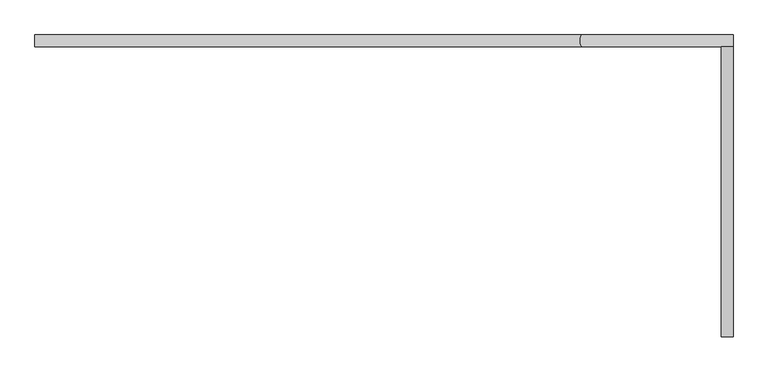
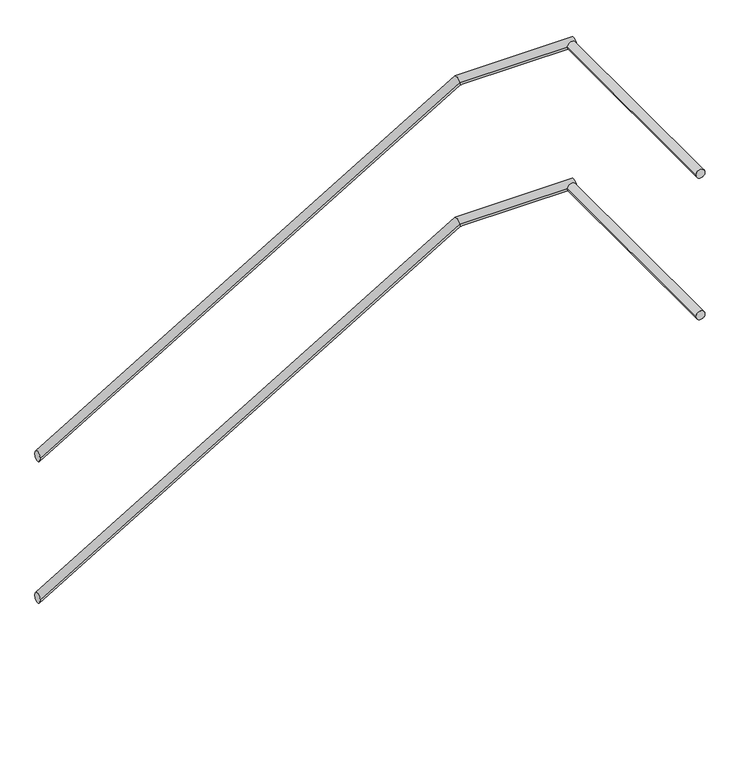
"""IFC4 building model written with IfcOpenShell, lengths in millimetres: railing geometry."""

from ifc_helpers import new_model, si_unit, frame, origin, place, context, project, spatial, circle_curve, ellipse_curve, source, transform, mapped, element, save
from ifc_brep_helpers import plane_surface, cylinder_surface, advanced_brep


def railing_5d0a0082(model_context):
    return source(origin(), model_context, "Body", "AdvancedBrep", [
        advanced_brep(
        [(43964.6, 23749.5208589, 1734.9618634), (43994.6, 23749.5208589, 1734.9618634), (43964.6, 24494.1208589, 1734.9618634), (43994.6, 24494.1208589, 1734.9618634)],
        [
            (0, 1, circle_curve(frame((43979.6, 23749.5208589, 1734.9618634), z_axis=(0.0, -1.0, 0.0), x_axis=(1.0, 0.0, 0.0)), 15.0)),
            (1, 0, circle_curve(frame((43979.6, 23749.5208589, 1734.9618634), z_axis=(0.0, -1.0, 0.0), x_axis=(1.0, 0.0, 0.0)), 15.0)),
            (2, 3, circle_curve(frame((43979.6, 24494.1208589, 1734.9618634), z_axis=(0.0, 1.0, 0.0), x_axis=(1.0, 0.0, 0.0)), 15.0)),
            (3, 2, circle_curve(frame((43979.6, 24494.1208589, 1734.9618634), z_axis=(0.0, 1.0, 0.0), x_axis=(1.0, 0.0, 0.0)), 15.0)),
            (0, 2),
            (3, 1),
        ],
        [
            plane_surface(frame((43979.6, 23749.5208589, 1749.9618634), z_axis=(0.0, -1.0, 0.0), x_axis=(0.0, 0.0, 1.0))),
            plane_surface(frame((43979.6, 24494.1208589, 1749.9618634), z_axis=(0.0, 1.0, 0.0), x_axis=(0.0, 0.0, 1.0))),
            cylinder_surface(frame((43979.6, 23749.5208589, 1734.9618634), z_axis=(0.0, -1.0, 0.0), x_axis=(1.0, 0.0, 0.0)), 15.0),
        ],
        [
            (0, [[1, 2]]),
            (1, [[3, 4]]),
            (2, [[-1, 5, -4, 6]]),
            (2, [[-2, -6, -3, -5]]),
        ],
    ),
        advanced_brep(
        [(43994.6, 24494.1208589, 1734.9618634), (43994.6, 24524.1208589, 1734.9618634), (43606.242552, 24494.1208589, 1734.9618634), (43606.242552, 24524.1208589, 1734.9618634), (42202.1161135, 24494.1208589, 899.1723166), (42202.1161135, 24524.1208589, 899.1723166)],
        [
            (0, 1, circle_curve(frame((43994.6, 24509.1208589, 1734.9618634), z_axis=(1.0, 0.0, 0.0), x_axis=(0.0, 1.0, 0.0)), 15.0)),
            (1, 0, circle_curve(frame((43994.6, 24509.1208589, 1734.9618634), z_axis=(1.0, 0.0, 0.0), x_axis=(0.0, 1.0, 0.0)), 15.0)),
            (0, 2),
            (2, 3, ellipse_curve(frame((43606.242552, 24509.1208589, 1734.9618634), z_axis=(0.9641817474962143, 0.0, 0.26524245096731114), x_axis=(0.265242450967311, 0.0, -0.9641817474962145)), 15.5572329, 15.0)),
            (3, 1),
            (3, 2, ellipse_curve(frame((43606.242552, 24509.1208589, 1734.9618634), z_axis=(0.9641817474962143, 0.0, 0.26524245096731114), x_axis=(0.265242450967311, 0.0, -0.9641817474962145)), 15.5572329, 15.0)),
            (4, 5, ellipse_curve(frame((42202.1161135, 24509.1208589, 899.1723166), z_axis=(-1.0, 0.0, 0.0), x_axis=(0.0, 0.0, 1.0)), 17.4562134, 15.0)),
            (5, 4, ellipse_curve(frame((42202.1161135, 24509.1208589, 899.1723166), z_axis=(-1.0, 0.0, 0.0), x_axis=(0.0, 0.0, 1.0)), 17.4562134, 15.0)),
            (2, 4),
            (5, 3),
        ],
        [
            plane_surface(frame((43994.6, 24509.1208589, 1749.9618634), z_axis=(1.0, 0.0, 0.0), x_axis=(0.0, -1.0, 0.0))),
            cylinder_surface(frame((43994.6, 24509.1208589, 1734.9618634), z_axis=(1.0, 0.0, 0.0), x_axis=(0.0, 1.0, 0.0)), 15.0),
            plane_surface(frame((42202.1161135, 24509.1208589, 916.62853), z_axis=(-1.0, 0.0, 0.0), x_axis=(0.0, -1.0, 0.0))),
            cylinder_surface(frame((43609.7883714, 24509.1208589, 1737.0724701), z_axis=(0.8592928844097072, 0.0, 0.511483859767682), x_axis=(0.0, 1.0, 0.0)), 15.0),
        ],
        [
            (0, [[1, 2]]),
            (1, [[-1, 3, 4, 5]]),
            (1, [[-2, -5, 6, -3]]),
            (2, [[7, 8]]),
            (3, [[-4, 9, -8, 10]]),
            (3, [[-6, -10, -7, -9]]),
        ],
    ),
        advanced_brep(
        [(43964.6, 23749.5208589, 2234.9618634), (43994.6, 23749.5208589, 2234.9618634), (43964.6, 24494.1208589, 2234.9618634), (43994.6, 24494.1208589, 2234.9618634)],
        [
            (0, 1, circle_curve(frame((43979.6, 23749.5208589, 2234.9618634), z_axis=(0.0, -1.0, 0.0), x_axis=(1.0, 0.0, 0.0)), 15.0)),
            (1, 0, circle_curve(frame((43979.6, 23749.5208589, 2234.9618634), z_axis=(0.0, -1.0, 0.0), x_axis=(1.0, 0.0, 0.0)), 15.0)),
            (2, 3, circle_curve(frame((43979.6, 24494.1208589, 2234.9618634), z_axis=(0.0, 1.0, 0.0), x_axis=(1.0, 0.0, 0.0)), 15.0)),
            (3, 2, circle_curve(frame((43979.6, 24494.1208589, 2234.9618634), z_axis=(0.0, 1.0, 0.0), x_axis=(1.0, 0.0, 0.0)), 15.0)),
            (0, 2),
            (3, 1),
        ],
        [
            plane_surface(frame((43979.6, 23749.5208589, 2249.9618634), z_axis=(0.0, -1.0, 0.0), x_axis=(0.0, 0.0, 1.0))),
            plane_surface(frame((43979.6, 24494.1208589, 2249.9618634), z_axis=(0.0, 1.0, 0.0), x_axis=(0.0, 0.0, 1.0))),
            cylinder_surface(frame((43979.6, 23749.5208589, 2234.9618634), z_axis=(0.0, -1.0, 0.0), x_axis=(1.0, 0.0, 0.0)), 15.0),
        ],
        [
            (0, [[1, 2]]),
            (1, [[3, 4]]),
            (2, [[-1, 5, -4, 6]]),
            (2, [[-2, -6, -3, -5]]),
        ],
    ),
        advanced_brep(
        [(43994.6, 24494.1208589, 2234.9618634), (43994.6, 24524.1208589, 2234.9618634), (43606.242552, 24494.1208589, 2234.9618634), (43606.242552, 24524.1208589, 2234.9618634), (42202.1161135, 24494.1208589, 1399.1723166), (42202.1161135, 24524.1208589, 1399.1723166)],
        [
            (0, 1, circle_curve(frame((43994.6, 24509.1208589, 2234.9618634), z_axis=(1.0, 0.0, 0.0), x_axis=(0.0, 1.0, 0.0)), 15.0)),
            (1, 0, circle_curve(frame((43994.6, 24509.1208589, 2234.9618634), z_axis=(1.0, 0.0, 0.0), x_axis=(0.0, 1.0, 0.0)), 15.0)),
            (0, 2),
            (2, 3, ellipse_curve(frame((43606.242552, 24509.1208589, 2234.9618634), z_axis=(0.9641817474962143, 0.0, 0.26524245096731114), x_axis=(0.265242450967311, 0.0, -0.9641817474962145)), 15.5572329, 15.0)),
            (3, 1),
            (3, 2, ellipse_curve(frame((43606.242552, 24509.1208589, 2234.9618634), z_axis=(0.9641817474962143, 0.0, 0.26524245096731114), x_axis=(0.265242450967311, 0.0, -0.9641817474962145)), 15.5572329, 15.0)),
            (4, 5, ellipse_curve(frame((42202.1161135, 24509.1208589, 1399.1723166), z_axis=(-1.0, 0.0, 0.0), x_axis=(0.0, 0.0, 1.0)), 17.4562134, 15.0)),
            (5, 4, ellipse_curve(frame((42202.1161135, 24509.1208589, 1399.1723166), z_axis=(-1.0, 0.0, 0.0), x_axis=(0.0, 0.0, 1.0)), 17.4562134, 15.0)),
            (2, 4),
            (5, 3),
        ],
        [
            plane_surface(frame((43994.6, 24509.1208589, 2249.9618634), z_axis=(1.0, 0.0, 0.0), x_axis=(0.0, -1.0, 0.0))),
            cylinder_surface(frame((43994.6, 24509.1208589, 2234.9618634), z_axis=(1.0, 0.0, 0.0), x_axis=(0.0, 1.0, 0.0)), 15.0),
            plane_surface(frame((42202.1161135, 24509.1208589, 1416.62853), z_axis=(-1.0, 0.0, 0.0), x_axis=(0.0, -1.0, 0.0))),
            cylinder_surface(frame((43609.7883714, 24509.1208589, 2237.0724701), z_axis=(0.8592928844097072, 0.0, 0.511483859767682), x_axis=(0.0, 1.0, 0.0)), 15.0),
        ],
        [
            (0, [[1, 2]]),
            (1, [[-1, 3, 4, 5]]),
            (1, [[-2, -5, 6, -3]]),
            (2, [[7, 8]]),
            (3, [[-4, 9, -8, 10]]),
            (3, [[-6, -10, -7, -9]]),
        ],
    ),
    ])


if __name__ == "__main__":
    model = new_model("IFC4")
    model_context = context("Model", 3, world=origin())
    ifc_project = project(units=[si_unit("LENGTHUNIT", "METRE", prefix="MILLI")], contexts=[model_context])
    site = spatial("IfcSite", under=ifc_project)
    building = spatial("IfcBuilding", under=site)
    placement = place(None, origin())
    railing_shape = railing_5d0a0082(model_context)
    element("IfcRailing", 1, at=placement, inside=building, context=model_context, shape_type="MappedRepresentation", body=[
        mapped(railing_shape, transform((0.0, 0.0, 0.0), x_axis=(1.0, 0.0, 0.0), y_axis=(0.0, 1.0, 0.0), z_axis=(0.0, 0.0, 1.0))),
    ])
    save(model, "model.ifc")
